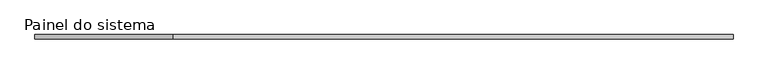
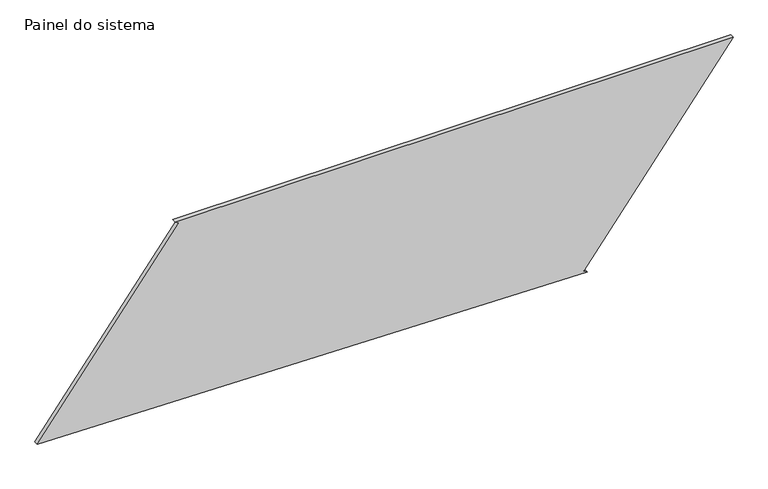
"""IFC4 building model written with IfcOpenShell, lengths in millimetres: plate geometry, Painel do sistema : Envidraçado."""

from ifc_helpers import new_model, si_unit, frame, origin, place, context, project, spatial, polyline, outline, extrude, source, transform, mapped, element, save


def painel_do_sistema_8dfcaf45(model_context):
    return source(origin(), model_context, "Body", "SweptSolid", [
        extrude(outline(polyline([(0.0, 1162.6830601), (15.2063352, 1142.8394876), (1136.6078664, 2002.1810952), (1136.6078664, -1207.4588688), (1121.4015312, -1187.6152963), (58.4303844, -2002.1810952), (0.0, 1162.6830601)])), frame((0.0, 24.5, 0.0), z_axis=(0.0, 1.0, 0.0), x_axis=(0.0, 0.0, 1.0)), (0.0, 0.0, 1.0), 25.0),
    ])


if __name__ == "__main__":
    model = new_model("IFC4")
    model_context = context("Model", 3, world=origin())
    ifc_project = project(units=[si_unit("LENGTHUNIT", "METRE", prefix="MILLI")], contexts=[model_context])
    site = spatial("IfcSite", under=ifc_project)
    building = spatial("IfcBuilding", under=site)
    placement = place(None, origin())
    painel_do_sistema_shape = painel_do_sistema_8dfcaf45(model_context)
    element("IfcPlate", 1, ObjectType="Painel do sistema : Envidraçado", at=placement, inside=building, context=model_context, shape_type="MappedRepresentation", body=[
        mapped(painel_do_sistema_shape, transform((0.0, 0.0, 0.0), x_axis=(1.0, 0.0, 0.0), y_axis=(0.0, 1.0, 0.0), z_axis=(0.0, 0.0, 1.0))),
    ])
    save(model, "model.ifc")

# Revit data of these elements
# Type "Painel do sistema : Envidraçado"
#   Construction Type Id = "GSP4R"
#   Analytic Construction = "Vidraça única Pilkington 1/8 pol"
#   Visual Light Transmittance = 0.9
#   Solar Heat Gain Coefficient = 0.86
#   Heat Transfer Coefficient (U) = 6.7069 W/(m²·K)
# Element 1 (IfcPlate, "Painel do sistema : Envidraçado")
#   Materials on its faces: "Vidro"
# Materials
#   "Vidro": class "Vidro", colour RGB 0 128 192, transparency 0.9, Description = "Vidro de sílica", Cost = 0
